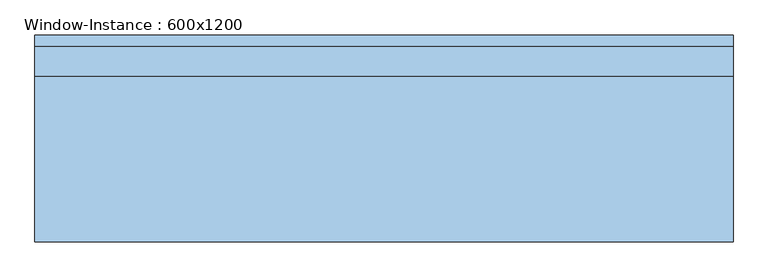
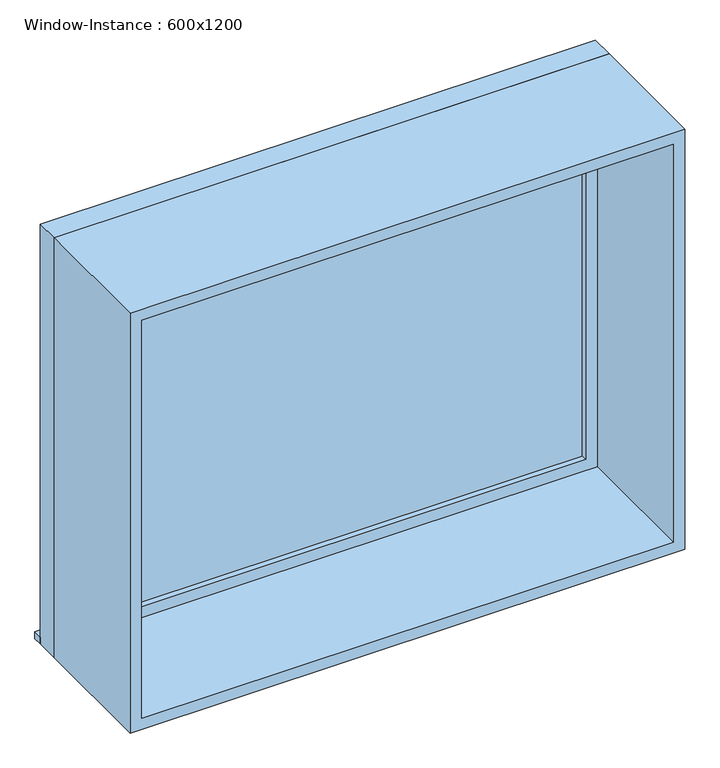
"""IFC4 building model written with IfcOpenShell, lengths in millimetres: window geometry, Window-Instance : 600x1200."""

from ifc_helpers import new_model, si_unit, frame, origin, place, context, project, spatial, polyline, outline, extrude, source, transform, mapped, element, save


def window_instance_600x1200_b3fcc358(model_context):
    return source(origin(), model_context, "Body", "SweptSolid", [
        extrude(outline(polyline([(-788.1, 235.4), (711.9, 235.4), (711.9, 210.0), (-788.1, 210.0), (-788.1, 235.4)])), frame((0.0, 0.0, 900.0), z_axis=(0.0, 0.0, 1.0), x_axis=(1.0, 0.0, 0.0)), (0.0, 0.0, 1.0), 19.05),
        extrude(outline(polyline([(648.4, 161.425), (-724.6, 161.425), (-724.6, 174.125), (648.4, 174.125), (648.4, 161.425)])), frame((0.0, 0.0, 963.5), z_axis=(0.0, 0.0, 1.0), x_axis=(1.0, 0.0, 0.0)), (0.0, 0.0, 1.0), 1073.0),
        extrude(outline(polyline([(2080.95, -769.05), (919.05, -769.05), (919.05, 692.85), (2080.95, 692.85), (2080.95, -769.05)]), holes=[polyline([(2036.5, -724.6), (2036.5, 648.4), (963.5, 648.4), (963.5, -724.6), (2036.5, -724.6)])]), frame((0.0, 145.55, 0.0), z_axis=(0.0, 1.0, 0.0), x_axis=(0.0, 0.0, 1.0)), (0.0, 0.0, 1.0), 44.45),
        extrude(outline(polyline([(2100.0, -788.1), (900.0, -788.1), (900.0, 711.9), (2100.0, 711.9), (2100.0, -788.1)]), holes=[polyline([(2068.25, -756.35), (2068.25, 680.15), (931.75, 680.15), (931.75, -756.35), (2068.25, -756.35)])]), frame((0.0, -210.0, 0.0), z_axis=(0.0, 1.0, 0.0), x_axis=(0.0, 0.0, 1.0)), (0.0, 0.0, 1.0), 355.55),
        extrude(outline(polyline([(2100.0, 711.9), (2100.0, -788.1), (900.0, -788.1), (900.0, 711.9), (2100.0, 711.9)]), holes=[polyline([(2080.95, 692.85), (919.05, 692.85), (919.05, -769.05), (2080.95, -769.05), (2080.95, 692.85)])]), frame((0.0, 145.55, 0.0), z_axis=(0.0, 1.0, 0.0), x_axis=(0.0, 0.0, 1.0)), (0.0, 0.0, 1.0), 64.45),
    ])


if __name__ == "__main__":
    model = new_model("IFC4")
    model_context = context("Model", 3, world=origin())
    ifc_project = project(units=[si_unit("LENGTHUNIT", "METRE", prefix="MILLI")], contexts=[model_context])
    site = spatial("IfcSite", under=ifc_project)
    building = spatial("IfcBuilding", under=site)
    placement = place(None, origin())
    window_instance_600x1200_shape = window_instance_600x1200_b3fcc358(model_context)
    element("IfcWindow", 1, ObjectType="Window-Instance : 600x1200", at=placement, inside=building, context=model_context, shape_type="MappedRepresentation", body=[
        mapped(window_instance_600x1200_shape, transform((0.0, 0.0, 0.0), x_axis=(1.0, 0.0, 0.0), y_axis=(0.0, 1.0, 0.0), z_axis=(0.0, 0.0, 1.0))),
    ])
    save(model, "model.ifc")

# Revit data of these elements
# Type "Window-Instance : 600x1200"
#   Type Mark = "7"
#   Construction Type Id = "GSP4R"
#   Assembly Code = "B2020100"
#   Analytic Construction = "1/8 in Pilkington single glazing"
#   Visual Light Transmittance = 0.9
#   Thermal Resistance (R) = 0.149095 (m²·K)/W
#   Solar Heat Gain Coefficient = 0.86
#   Heat Transfer Coefficient (U) = 6.70716 W/(m²·K)
#   Height [instance default] = 1200 mm
#   Default Sill Height = 900 mm
#   Width [instance default] = 600 mm
#   Window Inset = 20 mm
#   Glass Pane Material = WW-EC-GL-Storefront
#   Sash Material = WW-EC-RGB-White
#   Wall Closure = (empty or 0)
# Element 1 (IfcWindow, "Window-Instance : 600x1200")
#   Width = 1500 mm
#   Materials on its faces: "WW-EC-RGB-White", "WW-EC-GL-Storefront"
# Materials
#   "WW-EC-GL-Storefront": class "Glass", colour RGB 236 240 239, transparency 0.85, Description = "Storefront Glass", Cost = 0
#   "WW-EC-RGB-White": class "Generic", colour RGB 255 255 255, transparency 0, Comments = "If region requests off-white, swith asset color to RGB 231-228-220", Description = "Generic Color", Cost = 0
